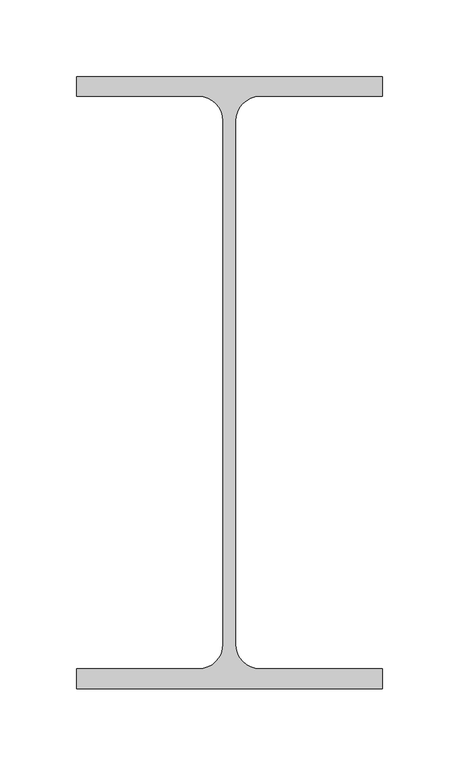
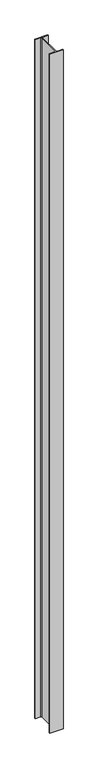
"""IFC4 building model written with IfcOpenShell, lengths in millimetres: column geometry, 0912_Steel Column_H_KSD3502 : H_SC_ASC_H-400x200x8x13."""

from ifc_helpers import new_model, si_unit, point, frame, frame_2d, origin, place, context, project, spatial, polyline, circle_curve, trimmed, segment, composite_curve, outline, extrude, source, transform, mapped, element, save


def column_a45a25b2(model_context):
    return source(origin(), model_context, "Body", "SweptSolid", [
        extrude(outline(composite_curve([segment(polyline([(100.0, 200.0), (100.0, 187.0), (20.0, 187.0)]), True, "CONTINUOUS"), segment(trimmed(circle_curve(frame_2d((20.0, 171.0)), 16.0), [point((20.0, 187.0))], [point((4.0, 171.0))], True, "CARTESIAN"), True, "CONTINUOUS"), segment(polyline([(4.0, 171.0), (4.0, -171.0)]), True, "CONTINUOUS"), segment(trimmed(circle_curve(frame_2d((20.0, -171.0)), 16.0), [point((4.0, -171.0))], [point((20.0, -187.0))], True, "CARTESIAN"), True, "CONTINUOUS"), segment(polyline([(20.0, -187.0), (100.0, -187.0), (100.0, -200.0), (-100.0, -200.0), (-100.0, -187.0), (-20.0, -187.0)]), True, "CONTINUOUS"), segment(trimmed(circle_curve(frame_2d((-20.0, -171.0)), 16.0), [point((-20.0, -187.0))], [point((-4.0, -171.0))], True, "CARTESIAN"), True, "CONTINUOUS"), segment(polyline([(-4.0, -171.0), (-4.0, 171.0)]), True, "CONTINUOUS"), segment(trimmed(circle_curve(frame_2d((-20.0, 171.0)), 16.0), [point((-4.0, 171.0))], [point((-20.0, 187.0))], True, "CARTESIAN"), True, "CONTINUOUS"), segment(polyline([(-20.0, 187.0), (-100.0, 187.0), (-100.0, 200.0), (100.0, 200.0)]), True, "CONTINUOUS")], self_intersect=False)), frame((0.0, 0.0, 6649.9720055), z_axis=(0.0, 0.0, 1.0), x_axis=(1.0, 0.0, 0.0)), (0.0, 0.0, 1.0), 11000.0),
    ])


if __name__ == "__main__":
    model = new_model("IFC4")
    model_context = context("Model", 3, world=origin())
    ifc_project = project(units=[si_unit("LENGTHUNIT", "METRE", prefix="MILLI")], contexts=[model_context])
    site = spatial("IfcSite", under=ifc_project)
    building = spatial("IfcBuilding", under=site)
    placement = place(None, origin())
    column_shape = column_a45a25b2(model_context)
    element("IfcColumn", 1, ObjectType="0912_Steel Column_H_KSD3502 : H_SC_ASC_H-400x200x8x13", at=placement, inside=building, context=model_context, shape_type="MappedRepresentation", body=[
        mapped(column_shape, transform((0.0, 0.0, 0.0), x_axis=(1.0, 0.0, 0.0), y_axis=(0.0, 1.0, 0.0), z_axis=(0.0, 0.0, 1.0))),
    ])
    save(model, "model.ifc")

# Revit data of these elements
# Type "0912_Steel Column_H_KSD3502 : H_SC_ASC_H-400x200x8x13"
#   H_WM Code_1 = "S01AA002-00001 | Main Steel Structure Fabrication Work | Shelter/Building | Medium Steel - Standard (90KG/M>Weight≥30KG/M) | Material: (   )"
#   H_WM Code_2 = "S03AA028-00001 | Main Steel Structure Erection Work | Shelter/Building | Medium Steel (90KG/M>Weight≥30KG/M) | Material: (   )"
#   H_WM Code_3 = "S01AA010-00001 | Main Steel Structure Fabrication Work | Shelter/Building | Steel Painting/Coating | for Non-Fireproofed Steel Surface, Surface Preparation, Primer, Second & Final Coat | Material: (   )"
#   H_Q'ty Cal Type Tag = "SC-Q2"
#   Width = 20.0 cm
#   Web Thickness = 0.8 cm
#   Web Fillet = 1.6 cm
#   Warping Constant = 648999.0 cm⁶
#   Torsional Moment of Inertia = 35.8981 cm⁴
#   Section Area = 84.12 cm²
#   Plastic Modulus weak axis = 268.0 cm³
#   Plastic Modulus strong axis = 1330.0 cm³
#   Perimeter = 1.56 m²/m
#   Nominal Weight = 66.00 kgf/m
#   Moment of Inertia weak axis = 1740.00 cm⁴
#   Moment of Inertia strong axis = 23700.00 cm⁴
#   Height = 40.0 cm
#   Flange Thickness = 1.3 cm
#   Elastic Modulus weak axis = 174.0 cm³
#   Elastic Modulus strong axis = 1190.0 cm³
#   Centroid Vertical = 20.0 cm
#   Centroid Horizontal = 10.0 cm
#   Structural Material [instance default] = Steel, 45-345
#   Section Name Key = ""
#   Bolt Spacing = 0
#   Assembly Code = ""
# Element 1 (IfcColumn, "0912_Steel Column_H_KSD3502 : H_SC_ASC_H-400x200x8x13")
#   Structural Material = none
# Materials
#   "Steel, 45-345": class "Metal", colour RGB 189 187 185, transparency 0, Description = "Steel 345 MPa", Cost = 0
